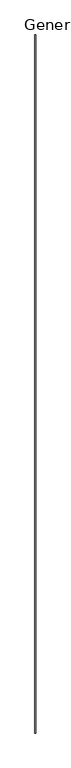
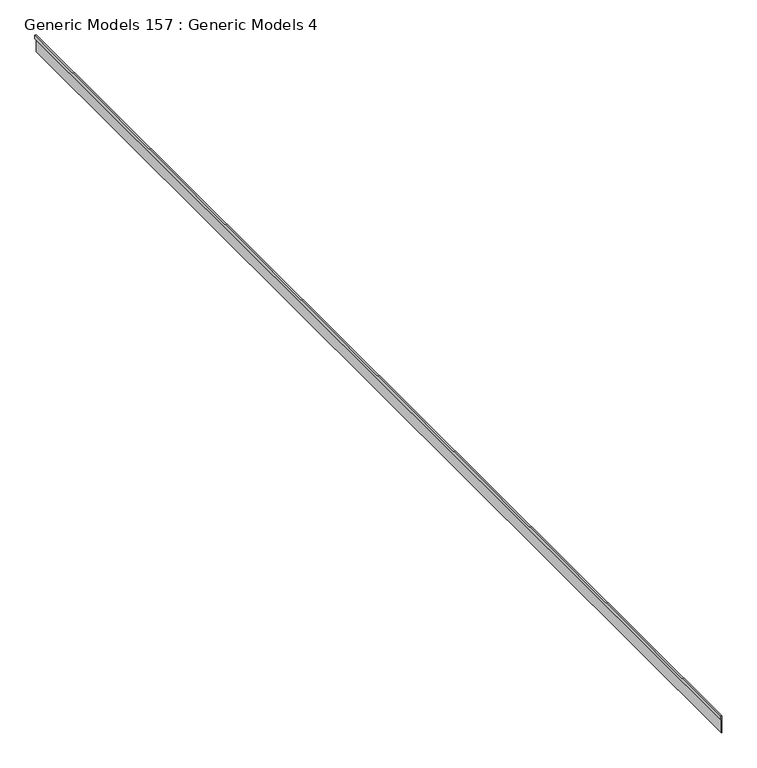
"""IFC4 building model written with IfcOpenShell, lengths in millimetres: proxy geometry, Generic Models 157 : Generic Models 4."""

from ifc_helpers import new_model, si_unit, origin, place, context, project, spatial, faceted_brep, source, transform, mapped, element, save


def generic_models_157_generic_models_4_33a7fcfd(model_context):
    return source(origin(), model_context, "Body", "Brep", [
        faceted_brep([(-10236.1097239, -5493.3230338, 122631.7984874), (-10236.1097239, -5493.3230338, 122793.7234874), (-10237.6972239, -5493.3230338, 122793.7234874), (-10237.6972239, -5493.3230338, 122820.8249647), (-10252.9339552, -5493.3230338, 122820.8249647), (-10252.9339552, -5493.3230338, 122793.7234874), (-10252.9339552, -5493.3230338, 122784.1984874), (-10239.2847239, -5493.3230338, 122784.1984874), (-10239.2847239, -5493.3230338, 122631.7984874), (-10252.9339552, 7054.2769662, 122820.8249648), (-10237.6972239, 7054.2769662, 122820.8249648), (-10237.6972239, 7054.2769662, 122793.7234874), (-10236.1097239, 7054.2769662, 122793.7234874), (-10236.1097239, 7054.2769662, 122631.7984874), (-10239.2847239, 7054.2769662, 122631.7984874), (-10239.2847239, 7054.2769662, 122784.1984874), (-10252.9339552, 7054.2769662, 122784.1984874), (-10252.9339552, 7054.2769662, 122793.7234874)], [[[0, 1, 2, 3, 4, 5, 6, 7, 8]], [[9, 10, 11, 12, 13, 14, 15, 16, 17]], [[4, 9, 17, 16, 6, 5]], [[13, 0, 8, 14]], [[0, 13, 12, 1]], [[9, 4, 3, 10]], [[2, 11, 10, 3]], [[11, 2, 1, 12]], [[7, 15, 14, 8]], [[15, 7, 6, 16]]]),
    ])


if __name__ == "__main__":
    model = new_model("IFC4")
    model_context = context("Model", 3, world=origin())
    ifc_project = project(units=[si_unit("LENGTHUNIT", "METRE", prefix="MILLI")], contexts=[model_context])
    site = spatial("IfcSite", under=ifc_project)
    building = spatial("IfcBuilding", under=site)
    placement = place(None, origin())
    generic_models_157_generic_models_4_shape = generic_models_157_generic_models_4_33a7fcfd(model_context)
    element("IfcBuildingElementProxy", 1, Name="Generic Models 157 : Generic Models 4", ObjectType="Generic Models 157 : Generic Models 4", at=placement, inside=building, context=model_context, shape_type="MappedRepresentation", body=[
        mapped(generic_models_157_generic_models_4_shape, transform((0.0, 0.0, 0.0), x_axis=(1.0, 0.0, 0.0), y_axis=(0.0, 1.0, 0.0), z_axis=(0.0, 0.0, 1.0))),
    ])
    save(model, "model.ifc")

# Revit data of these elements
# Element 1 (IfcBuildingElementProxy, "Generic Models 157 : Generic Models 4")
#   Materials on its faces: "_MORTAR SETTING BED"
# Materials
#   "_MORTAR SETTING BED": class "Generic", colour RGB 191 191 191, transparency 0, Cost = 0
